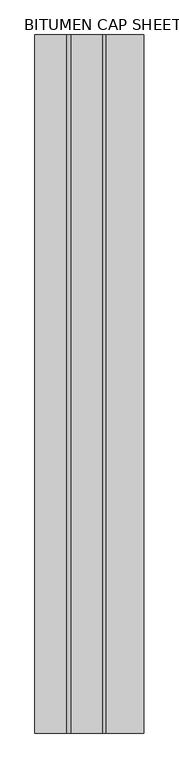
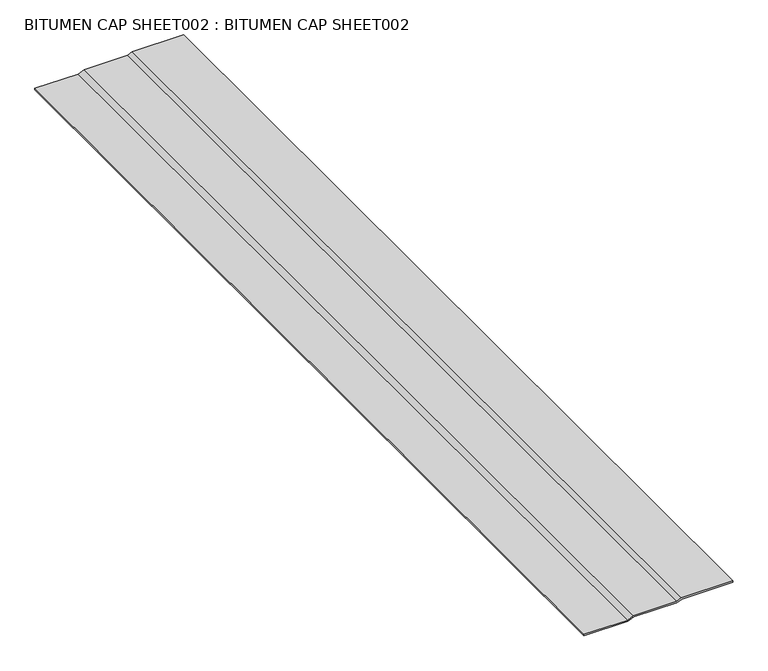
"""IFC4 building model written with IfcOpenShell, lengths in millimetres: proxy geometry, BITUMEN CAP SHEET002 : BITUMEN CAP SHEET002."""

from ifc_helpers import new_model, si_unit, frame, origin, place, context, project, spatial, polyline, outline, extrude, source, transform, mapped, element, save


def bitumen_cap_sheet002_bitumen_cap_sheet002_cc5fe4d3(model_context):
    return source(origin(), model_context, "Body", "SweptSolid", [
        extrude(outline(polyline([(40259.2002678, -4699.8063764), (40259.2002678, -4607.6417148), (40264.4862773, -4595.1768962), (40264.4862773, -4504.46274), (40268.8188423, -4494.7463535), (40268.8188423, -4387.5351424), (40271.9940719, -4387.5351424), (40271.9940719, -4495.421639), (40267.6612773, -4505.1385405), (40267.6612773, -4595.8222961), (40262.3752678, -4608.2871148), (40262.3752678, -4699.8063764), (40259.2002678, -4699.8063764)])), frame((0.0, -1052.8906574, 0.0), z_axis=(0.0, 1.0, 0.0), x_axis=(0.0, 0.0, 1.0)), (0.0, 0.0, 1.0), 2000.25),
    ])


if __name__ == "__main__":
    model = new_model("IFC4")
    model_context = context("Model", 3, world=origin())
    ifc_project = project(units=[si_unit("LENGTHUNIT", "METRE", prefix="MILLI")], contexts=[model_context])
    site = spatial("IfcSite", under=ifc_project)
    building = spatial("IfcBuilding", under=site)
    placement = place(None, origin())
    bitumen_cap_sheet002_bitumen_cap_sheet002_shape = bitumen_cap_sheet002_bitumen_cap_sheet002_cc5fe4d3(model_context)
    element("IfcBuildingElementProxy", 1, Name="BITUMEN CAP SHEET002 : BITUMEN CAP SHEET002", ObjectType="BITUMEN CAP SHEET002 : BITUMEN CAP SHEET002", at=placement, inside=building, context=model_context, shape_type="MappedRepresentation", body=[
        mapped(bitumen_cap_sheet002_bitumen_cap_sheet002_shape, transform((0.0, 0.0, 0.0), x_axis=(1.0, 0.0, 0.0), y_axis=(0.0, 1.0, 0.0), z_axis=(0.0, 0.0, 1.0))),
    ])
    save(model, "model.ifc")

# Revit data of these elements
# Type "BITUMEN CAP SHEET002 : BITUMEN CAP SHEET002"
#   NameOverride = "BITUMEN CAP SHEET002"
# Element 1 (IfcBuildingElementProxy, "BITUMEN CAP SHEET002 : BITUMEN CAP SHEET002")
#   Materials on its faces: "MODIFIED BITUMEN GRANULE SURFACED CAP SHEET"
# Materials
#   "MODIFIED BITUMEN GRANULE SURFACED CAP SHEET": class "Unassigned", colour RGB 85 85 127, transparency 0
